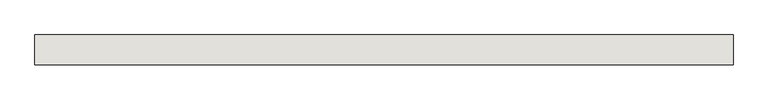
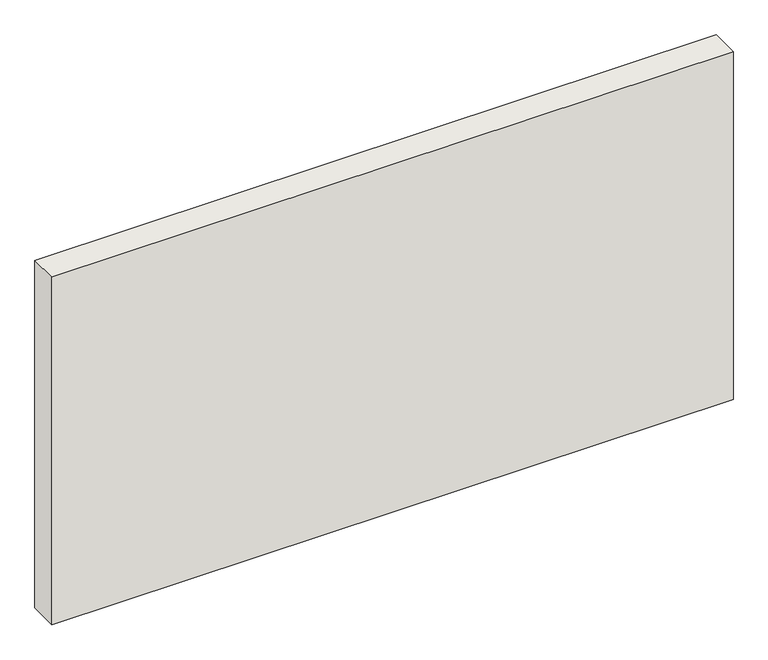
"""IFC4 building model written with IfcOpenShell, lengths in millimetres: wall geometry, Holzwand."""

from ifc_helpers import new_model, si_unit, origin, origin_with_axes, place, context, project, spatial, polyline, outline, extrude, source, transform, mapped, element, save


def wall_b3714669(model_context):
    return source(origin(), model_context, "Body", "SweptSolid", [
        extrude(outline(polyline([(0.0, 200.0), (4650.0, 200.0), (4650.0, 0.0), (0.0, 0.0), (0.0, 200.0)])), origin_with_axes(), (0.0, 0.0, 1.0), 2510.0),
    ])


if __name__ == "__main__":
    model = new_model("IFC4")
    model_context = context("Model", 3, world=origin())
    ifc_project = project(units=[si_unit("LENGTHUNIT", "METRE", prefix="MILLI")], contexts=[model_context])
    site = spatial("IfcSite", under=ifc_project)
    building = spatial("IfcBuilding", under=site)
    placement = place(None, origin())
    wall_shape = wall_b3714669(model_context)
    element("IfcWall", 1, ObjectType="Holzwand", at=placement, inside=building, context=model_context, shape_type="MappedRepresentation", body=[
        mapped(wall_shape, transform((0.0, 0.0, 0.0), x_axis=(1.0, 0.0, 0.0), y_axis=(0.0, 1.0, 0.0), z_axis=(0.0, 0.0, 1.0))),
    ])
    save(model, "model.ifc")

# Revit data of these elements
# Element 1 (IfcWall, "Holzwand")
#   Materials on its faces: "holzschalung"
# Materials
#   "holzschalung": class "Unassigned", colour RGB 128 128 128, transparency 0
